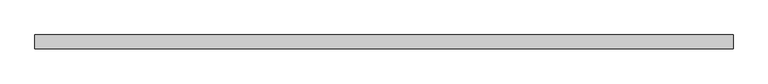
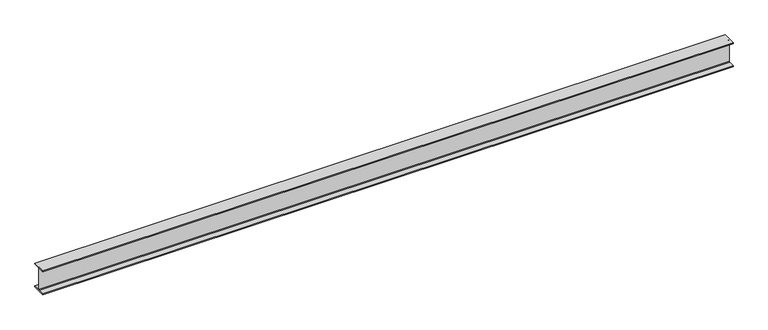
"""IFC4 building model written with IfcOpenShell, lengths in millimetres: beam geometry, Old_Steel Beam_H-KSD3502 : H_SB_ASB_H-340×250x9x14."""

from ifc_helpers import new_model, si_unit, point, frame, frame_2d, origin, place, context, project, spatial, polyline, circle_curve, trimmed, segment, composite_curve, outline, extrude, source, transform, mapped, element, save


def beam_bba65be6(model_context):
    return source(origin(), model_context, "Body", "SweptSolid", [
        extrude(outline(composite_curve([segment(polyline([(82.5, -141.5), (82.5, -151.7), (-82.5, -151.7), (-82.5, -141.5), (-11.9, -141.5)]), True, "CONTINUOUS"), segment(trimmed(circle_curve(frame_2d((-11.9, -132.6)), 8.9), [point((-11.9, -141.5))], [point((-3.0, -132.6))], True, "CARTESIAN"), True, "CONTINUOUS"), segment(polyline([(-3.0, -132.6), (-3.0, 132.6)]), True, "CONTINUOUS"), segment(trimmed(circle_curve(frame_2d((-11.9, 132.6)), 8.9), [point((-3.0, 132.6))], [point((-11.9, 141.5))], True, "CARTESIAN"), True, "CONTINUOUS"), segment(polyline([(-11.9, 141.5), (-82.5, 141.5), (-82.5, 151.7), (82.5, 151.7), (82.5, 141.5), (11.9, 141.5)]), True, "CONTINUOUS"), segment(trimmed(circle_curve(frame_2d((11.9, 132.6)), 8.9), [point((11.9, 141.5))], [point((3.0, 132.6))], True, "CARTESIAN"), True, "CONTINUOUS"), segment(polyline([(3.0, 132.6), (3.0, -132.6)]), True, "CONTINUOUS"), segment(trimmed(circle_curve(frame_2d((11.9, -132.6)), 8.9), [point((3.0, -132.6))], [point((11.9, -141.5))], True, "CARTESIAN"), True, "CONTINUOUS"), segment(polyline([(11.9, -141.5), (82.5, -141.5)]), True, "CONTINUOUS")], self_intersect=False)), frame((-4087.3, 0.0, 0.0), z_axis=(1.0, 0.0, 0.0), x_axis=(0.0, 1.0, 0.0)), (0.0, 0.0, 1.0), 8337.3),
    ])


if __name__ == "__main__":
    model = new_model("IFC4")
    model_context = context("Model", 3, world=origin())
    ifc_project = project(units=[si_unit("LENGTHUNIT", "METRE", prefix="MILLI")], contexts=[model_context])
    site = spatial("IfcSite", under=ifc_project)
    building = spatial("IfcBuilding", under=site)
    placement = place(None, origin())
    beam_shape = beam_bba65be6(model_context)
    element("IfcBeam", 1, ObjectType="Old_Steel Beam_H-KSD3502 : H_SB_ASB_H-340×250x9x14", at=placement, inside=building, context=model_context, shape_type="MappedRepresentation", body=[
        mapped(beam_shape, transform((0.0, 0.0, 0.0), x_axis=(1.0, 0.0, 0.0), y_axis=(0.0, 1.0, 0.0), z_axis=(0.0, 0.0, 1.0))),
    ])
    save(model, "model.ifc")

# Revit data of these elements
# Type "Old_Steel Beam_H-KSD3502 : H_SB_ASB_H-340×250x9x14"
#   Width = 25.0 cm
#   Web Thickness = 0.9 cm
#   Web Fillet = 2.0 cm
#   Warping Constant = 968661.0 cm⁶
#   Torsional Moment of Inertia = 53.6551 cm⁴
#   Torsional Modulus = 1.0 cm³
#   Section Area = 101.5 cm²
#   Plastic Modulus weak axis = 447.0 cm³
#   Plastic Modulus strong axis = 1410.0 cm³
#   Perimeter = 1.63 m²/m
#   Nominal Weight = 79.70 kgf/m
#   Moment of Inertia weak axis = 3650.00 cm⁴
#   Moment of Inertia strong axis = 21700.00 cm⁴
#   Height = 34.0 cm
#   Flange Thickness = 1.4 cm
#   Elastic Modulus weak axis = 292.0 cm³
#   Elastic Modulus strong axis = 1280.0 cm³
#   Centroid Vertical = 17.0 cm
#   Centroid Horizontal = 12.5 cm
#   Length [instance default] = 1.5240 m
#   Structural Material [instance default] = Steel, 45-345
#   Assembly Code = ""
# Element 1 (IfcBeam, "Old_Steel Beam_H-KSD3502 : H_SB_ASB_H-340×250x9x14")
#   Structural Material = none
# Materials
#   "Steel, 45-345": class "Metal", colour RGB 189 187 185, transparency 0, Description = "Steel 345 MPa", Cost = 0
